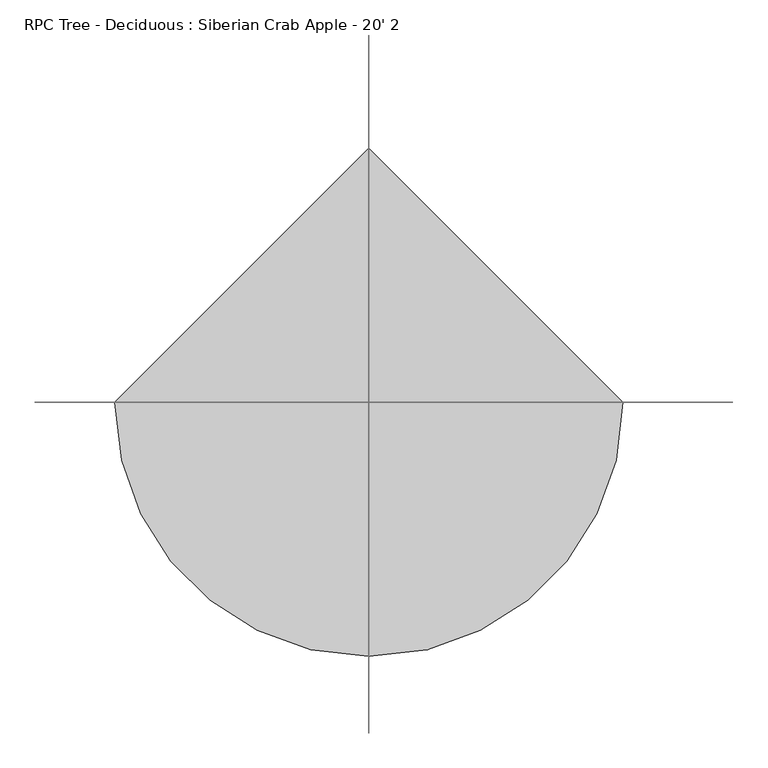
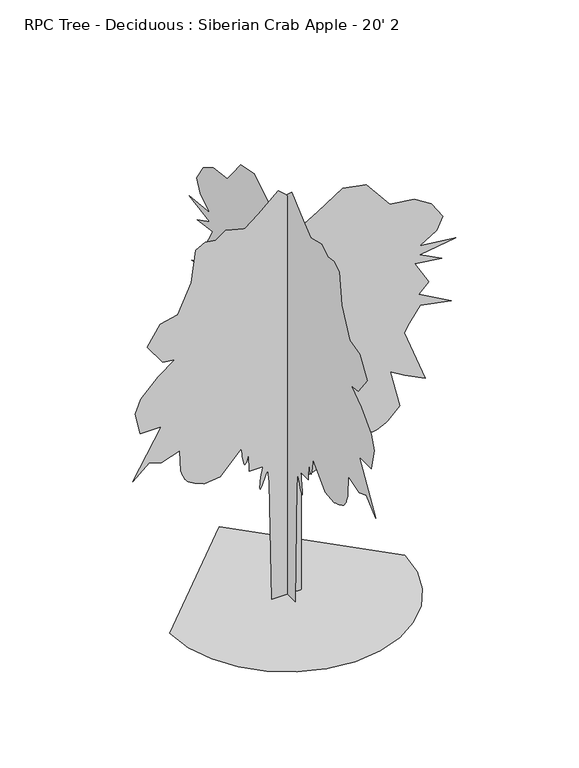
"""IFC4 building model written with IfcOpenShell, lengths in millimetres: geographic element geometry, RPC Tree - Deciduous : Siberian Crab Apple - 20' 2."""

from ifc_helpers import new_model, si_unit, origin, place, context, project, spatial, triangles, source, transform, mapped, element, save


def rpc_tree_deciduous_siberian_crab_apple_20_2_052c092b(model_context):
    return source(origin(), model_context, "Body", "Tessellation", [
        triangles([(-0.5602972, -201.7007698, 0.1401761), (-0.5602953, -233.6267644, 1770.9888485), (-0.560294, -257.4323607, 1961.4323112), (-0.5602928, -281.0760302, 1899.1069004), (-0.5602909, -303.7481383, 1840.3247326), (-0.5602896, -324.477142, 1788.6165516), (-0.560289, -342.2908439, 1747.5319954), (-0.5602877, -356.2177191, 1720.6015171), (-0.5602877, -365.2868239, 1711.3685051), (-0.5602871, -368.5253254, 1723.3764931), (-0.5602871, -367.3690006, 1751.3483322), (-0.5602877, -364.1298451, 1786.8131733), (-0.5602877, -359.1558755, 1828.5264702), (-0.5602883, -352.7938002, 1875.2308868), (-0.560289, -345.3909453, 1925.6881268), (-0.560289, -337.2934018, 1978.6472488), (-0.5602896, -328.8491498, 2032.8510624), (-0.5602782, -519.2951197, 2032.8510624), (-0.5602775, -527.2301368, 2286.7756794), (-0.5602769, -537.409203, 2251.45051), (-0.5602763, -547.4498692, 2218.4176426), (-0.5602763, -557.212391, 2189.9568798), (-0.5602756, -566.5589862, 2168.3731682), (-0.560275, -575.3505644, 2155.95256), (-0.5602744, -583.4474902, 2154.9809624), (-0.5602737, -590.7119087, 2167.7508224), (-0.5602737, -597.2822926, 2191.1633469), (-0.5602731, -603.4360957, 2219.9861515), (-0.5602731, -609.2431904, 2253.3237968), (-0.5602724, -614.7721407, 2290.2745937), (-0.5602724, -620.0934729, 2329.9240631), (-0.5602718, -625.2757147, 2371.3833057), (-0.5602718, -630.3881207, 2413.7443829), (-0.560254, -931.9290173, 2096.3322166), (-0.5602407, -1154.1161819, 2072.5259663), (-0.5602375, -1198.140893, 2089.5313236), (-0.560235, -1241.0543346, 2106.536681), (-0.5602331, -1281.7453102, 2123.5420383), (-0.5602305, -1319.1087273, 2140.5410007), (-0.5602287, -1352.0336071, 2157.5463581), (-0.5602267, -1379.4022854, 2174.5517155), (-0.5602255, -1400.1033474, 2191.5570728), (-0.5602248, -1416.1815811, 2210.4102825), (-0.5602242, -1430.5961082, 2232.5973003), (-0.5602229, -1443.6200226, 2257.5592941), (-0.5602223, -1455.5389172, 2284.7436813), (-0.5602217, -1466.6197815, 2313.5917751), (-0.560221, -1477.1416683, 2343.5511383), (-0.5602204, -1487.3906067, 2374.063084), (-0.5602197, -1503.2656551, 2683.5376534), (-0.5602039, -1765.127869, 2596.2502487), (-0.5601937, -1939.7026783, 2659.7315483), (-0.5601798, -2169.8210449, 2453.4191414), (-0.5602039, -1765.127869, 3135.8495796), (-0.5601861, -2066.6648415, 3135.8495796), (-0.5601816, -2138.0835926, 3453.2552055), (-0.5601867, -2058.7273899, 3651.6364105), (-0.5602013, -1812.7403698, 3905.5610275), (-0.5602153, -1574.6780113, 4080.1419411), (-0.5602051, -1749.2528206, 4103.9419418), (-0.5601925, -1963.5087833, 4397.5478577), (-0.5602032, -1780.9965225, 4683.2161766), (-0.5602178, -1535.0031075, 4738.7598793), (-0.5602293, -1344.5596447, 5151.396611), (-0.5602331, -1281.0784904, 5619.5709412), (-0.5602407, -1146.1786577, 5690.9898376), (-0.5602496, -995.4101715, 5667.1837326), (-0.5602585, -852.5727419, 5770.3396454), (-0.5602744, -582.7769279, 5698.9271439), (-0.5602858, -392.3315758, 5849.6958481), (-0.5603029, -106.6631932, 6095.6895538), (-0.5603163, 115.523381, 5897.3080582), (-0.5603163, 115.523381, 5659.245845), (-0.5603245, 258.3569228, 5476.7401245), (-0.5603366, 456.7385456, 5587.8339249), (-0.5603575, 805.8874374, 5817.9518555), (-0.5603772, 1139.1682571, 5754.4708466), (-0.5603893, 1345.4803734, 5500.5462296), (-0.5603969, 1472.4490768, 5341.8402191), (-0.5604179, 1821.59855, 5294.228009), (-0.5604325, 2067.5919651, 5143.4593048), (-0.560442, 2226.2917259, 4897.4655991), (-0.5604369, 2139.0043213, 4722.8910805), (-0.5604223, 1900.9485031, 4572.1226669), (-0.5604528, 2408.8039867, 4516.5789642), (-0.5604223, 1900.9485031, 4437.2227615), (-0.5604407, 2210.4230724, 4278.5167511), (-0.5604185, 1829.529752, 4326.1292519), (-0.56043, 2027.9108116, 3984.9172302), (-0.5604217, 1885.0797043, 3850.0173248), (-0.560449, 2345.3228325, 3588.1551109), (-0.560423, 1908.8859547, 3675.4425156), (-0.5604134, 1750.1799442, 3461.1928024), (-0.560409, 1678.7611931, 3342.1616959), (-0.5604274, 1980.2983109, 2556.5753448), (-0.5604096, 1686.69879, 2699.4125565), (-0.5603976, 1480.3802788, 2826.374865), (-0.5604052, 1615.2800388, 2270.9070259), (-0.5603956, 1448.6428265, 2104.2696682), (-0.5603937, 1416.3657269, 2085.6895523), (-0.5603918, 1384.3044571, 2067.8777035), (-0.5603899, 1352.6559528, 2051.5900349), (-0.560388, 1321.6297943, 2037.5945229), (-0.5603861, 1291.441666, 2026.6534756), (-0.5603842, 1262.2887943, 2019.5223701), (-0.5603829, 1234.3931133, 2016.9824089), (-0.5603811, 1206.7197298, 2019.0651306), (-0.5603798, 1178.2208879, 2024.894426), (-0.5603779, 1149.0234695, 2033.8479492), (-0.5603759, 1119.2736139, 2045.297105), (-0.5603741, 1089.1046705, 2058.6257973), (-0.5603721, 1058.656311, 2073.1990356), (-0.5603702, 1028.0746748, 2088.3946198), (-0.5603702, 1019.444969, 2098.5293209), (-0.5603696, 1010.0533184, 2108.2448616), (-0.560369, 999.131238, 2117.1284763), (-0.5603677, 985.9231779, 2124.7675449), (-0.5603671, 969.6607985, 2130.7366573), (-0.5603658, 949.5756872, 2134.6229027), (-0.5603645, 924.918544, 2136.0071205), (-0.5603626, 892.850952, 2139.7092201), (-0.5603601, 852.0393442, 2150.0723957), (-0.5603569, 803.9443148, 2165.9919182), (-0.5603537, 750.0199173, 2186.3501232), (-0.5603506, 691.7204235, 2210.041991), (-0.5603467, 630.5036659, 2235.950148), (-0.5603429, 567.8315103, 2262.969429), (-0.5603372, 464.6735264, 2143.9447174), (-0.5603372, 464.6735264, 1945.5636578), (-0.5603404, 520.2190822, 1755.120195), (-0.560329, 329.7743477, 1691.6390408), (-0.560322, 218.6813649, 2001.1073605), (-0.5603233, 220.2409354, 0.0), (-1667.0454838, -6.4e-06, 0.5321514), (-1623.0016605, -381.6984675, 0.5321527), (-1497.5824265, -732.2271807, 0.5321565), (-1300.8143497, -1041.5430387, 0.5321622), (-1042.7559008, -1299.6078827, 0.5321698), (-733.4400427, -1496.3695644, 0.5321793), (-382.9106755, -1621.7887985, 0.5321895), (-1.2126887, -1665.8326218, 0.5322009), (380.4856055, -1621.7887985, 0.5322124), (731.0143187, -1496.3695644, 0.5322225), (1040.3301767, -1299.6014877, 0.532232), (1298.3950207, -1041.5430387, 0.5322396), (1495.1567024, -732.2271807, 0.5322454), (1620.5759365, -381.6978135, 0.5322492), (1664.6197598, 0.0001455, 0.5322505), (-1.2129808, 1665.8326218, 0.5322009), (-223.3549713, 0.0003636, 0.4735541), (-255.2809841, 0.0002642, 1771.3190609), (-279.0865623, 0.0002491, 1961.7689186), (-302.7302317, 0.0002561, 1899.4435078), (-325.4023398, 0.0002559, 1840.654945), (-346.1307258, 0.0002629, 1788.953159), (-363.9444277, 0.0002625, 1747.8622078), (-377.8719206, 0.000262, 1720.9317295), (-386.9404078, 0.0002688, 1711.7051125), (-390.1795269, 0.0002609, 1723.7129551), (-389.0225481, 0.0002601, 1751.6785446), (-385.7840466, 0.0002594, 1787.1433857), (-380.810077, 0.0002586, 1828.8566826), (-374.4480017, 0.0002577, 1875.5673489), (-367.0444928, 0.0002496, 1926.0247341), (-358.9476033, 0.0002487, 1978.9774612), (-350.5033513, 0.0002479, 2033.1812748), (-540.9487035, 0.0002455, 2033.1812748), (-548.8836843, 0.0002299, 2287.1122868), (-559.0634045, 0.00023, 2251.7871174), (-569.1034166, 0.0002374, 2218.747855), (-578.8665925, 0.0002374, 2190.2934872), (-588.2131877, 0.0002372, 2168.7097755), (-597.0041482, 0.0002368, 2156.2827724), (-605.1016917, 0.0002361, 2155.3111748), (-612.3654562, 0.0002351, 2168.0810349), (-618.9364941, 0.0002338, 2191.4935593), (-625.0902609, 0.0002324, 2220.3227589), (-630.8967379, 0.0002308, 2253.6602589), (-636.4244528, 0.0002293, 2290.6046608), (-641.745785, 0.0002276, 2330.2606705), (-646.9273727, 0.0002259, 2371.7135181), (-652.0391247, 0.0002242, 2414.0745953), (-953.5825647, 0.0002432, 2096.668824), (-1175.7697294, 0.0002459, 2072.8625736), (-1219.7944405, 0.0002415, 2089.861536), (-1262.7079548, 0.0002444, 2106.8668934), (-1303.398785, 0.0002403, 2123.8722507), (-1340.7623474, 0.0002364, 2140.8776081), (-1373.6872272, 0.0002403, 2157.8829655), (-1401.0557602, 0.0002373, 2174.8819279), (-1421.7568222, 0.000235, 2191.8872852), (-1437.8350559, 0.000233, 2210.7404949), (-1452.2495831, 0.000231, 2232.9275127), (-1465.2734974, 0.0002291, 2257.8893612), (-1477.1925373, 0.0002346, 2285.0738937), (-1488.2732563, 0.0002327, 2313.9219875), (-1498.7952885, 0.0002309, 2343.8813507), (-1509.0442268, 0.000229, 2374.3995461), (-1524.9192753, 0.0002038, 2683.8742607), (-1786.7814892, 0.0002122, 2596.5868561), (-1961.3561531, 0.0002093, 2660.067865), (-2191.4745197, 0.0002241, 2453.7493538), (-1786.7814892, 0.0001815, 3136.179792), (-2088.3184616, 0.0001838, 3136.179792), (-2159.7372128, 0.0001606, 3453.5918129), (-2080.3810101, 0.0001472, 3651.9730179), (-1834.3938446, 0.0001324, 3905.8976349), (-1596.3316315, 0.0001266, 4080.4721535), (-1770.9062954, 0.0001249, 4104.2785492), (-1985.1624035, 0.0001043, 4397.884465), (-1802.6501427, 9.02e-05, 4683.546389), (-1556.6567276, 8.13e-05, 4739.0964867), (-1366.2132648, 5.68e-05, 5151.7268234), (-1302.7321106, 3.4e-05, 5619.9075485), (-1167.8322052, 2.93e-05, 5691.326445), (-1017.063719, 2.89e-05, 5667.52034), (-874.226362, 2.4e-05, 5770.6762527), (-604.4311295, 2.83e-05, 5699.2573563), (-413.9851233, 1.89e-05, 5850.0260605), (-128.316768, 7e-07, 6096.0197662), (93.8691795, 1.91e-05, 5897.6382706), (93.8691795, 3.35e-05, 5659.5824524), (236.7027213, 4.44e-05, 5477.0703369), (435.0843441, 3.7e-05, 5588.1641373), (784.23389, 1.75e-05, 5818.2884628), (1117.5147097, 2.73e-05, 5754.8074539), (1323.8268986, 3.87e-05, 5500.876442), (1450.7954567, 4.75e-05, 5342.1704315), (1799.9450752, 5.09e-05, 5294.5646164), (2045.9320953, 6.28e-05, 5143.7895172), (2204.6381058, 7.7e-05, 4897.8022064), (2117.3508465, 8.9e-05, 4723.2276878), (1879.294883, 9.41e-05, 4572.4592743), (2387.1503666, 9.74e-05, 4516.9091766), (1879.294883, 0.0001055, 4437.5593689), (2188.7694523, 0.0001087, 4278.8533585), (1807.8761318, 0.0001097, 4326.4655685), (2006.2571915, 0.0001303, 3985.2474426), (1863.4262295, 0.0001361, 3850.3539322), (2323.6693577, 0.0001559, 3588.4853233), (1887.2323345, 0.0001508, 3675.7791229), (1728.5263241, 0.0001576, 3461.5230148), (1657.1077183, 0.0001693, 3342.4983032), (1958.6446907, 0.0002124, 2556.9119522), (1665.0451698, 0.0002038, 2699.7427689), (1458.7266586, 0.0001962, 2826.7050774), (1593.626564, 0.0002321, 2271.2434879), (1426.9892063, 0.0002441, 2104.5998806), (1394.7121067, 0.0002417, 2086.0261597), (1362.6508369, 0.0002467, 2068.2079159), (1331.0023327, 0.0002443, 2051.9264969), (1299.9761742, 0.0002493, 2037.9247353), (1269.7881912, 0.0002469, 2026.983688), (1240.6351742, 0.0002445, 2019.8589775), (1212.7332436, 0.0002494, 2017.3126213), (1185.0661823, 0.0002469, 2019.395343), (1156.5672678, 0.0002441, 2025.2246384), (1127.3699221, 0.0002486, 2034.1781616), (1097.6200665, 0.0002456, 2045.6337124), (1067.451123, 0.0002425, 2058.9560097), (1037.0027636, 0.0002466, 2073.529248), (1006.4210546, 0.0002434, 2088.7312271), (997.7914215, 0.0002424, 2098.8659283), (988.3996983, 0.0002412, 2108.581469), (977.4776905, 0.00024, 2117.4650837), (964.2696304, 0.0002386, 2125.0977573), (948.007251, 0.0002369, 2131.0668697), (927.9221397, 0.0002423, 2134.9529697), (903.2649965, 0.0002401, 2136.3437279), (871.1974045, 0.0002371, 2140.0456821), (830.3857967, 0.0002405, 2150.4090031), (782.2907673, 0.0002357, 2166.3221306), (728.3663698, 0.0002376, 2186.6803356), (670.066876, 0.0002389, 2210.3722034), (608.8494644, 0.0002327, 2236.28661), (546.1773088, 0.0002336, 2263.3060364), (443.0193249, 0.0002425, 2144.2749298), (443.0193249, 0.0002484, 1945.8938702), (498.5654984, 0.0002591, 1755.4504074), (308.1207639, 0.0002658, 1691.9692532), (197.0271634, 0.0002467, 2001.4438225), (198.5867339, 0.0003649, 0.3333907)], [[85, 84, 86], [53, 52, 54], [91, 90, 92], [87, 86, 88], [95, 94, 96], [96, 94, 97], [9, 8, 10], [52, 51, 54], [51, 50, 54], [1, 133, 2], [133, 132, 2], [2, 132, 3], [131, 130, 132], [130, 129, 132], [129, 128, 132], [18, 17, 19], [71, 70, 72], [72, 70, 73], [10, 8, 11], [8, 7, 11], [11, 7, 12], [7, 6, 12], [12, 6, 13], [6, 5, 13], [13, 5, 14], [5, 4, 14], [14, 4, 15], [4, 3, 15], [15, 3, 16], [16, 3, 17], [55, 54, 56], [89, 88, 90], [56, 54, 57], [57, 54, 58], [61, 60, 62], [62, 60, 63], [60, 59, 63], [25, 24, 26], [24, 23, 26], [26, 23, 27], [23, 22, 27], [27, 22, 28], [22, 21, 28], [28, 21, 29], [21, 20, 29], [29, 20, 30], [20, 19, 30], [30, 19, 31], [82, 81, 83], [83, 81, 84], [81, 80, 84], [80, 79, 84], [70, 69, 73], [98, 97, 99], [31, 19, 32], [99, 97, 100], [58, 54, 59], [100, 97, 101], [101, 97, 102], [102, 97, 103], [103, 97, 104], [104, 97, 105], [105, 97, 106], [106, 97, 107], [107, 97, 108], [108, 97, 109], [109, 97, 110], [110, 97, 111], [111, 97, 112], [112, 97, 113], [113, 97, 114], [114, 97, 115], [115, 97, 116], [116, 97, 117], [117, 97, 118], [118, 97, 119], [119, 97, 120], [120, 97, 121], [121, 97, 122], [122, 97, 123], [123, 97, 124], [124, 97, 125], [125, 97, 126], [126, 97, 127], [65, 64, 66], [66, 64, 67], [68, 67, 69], [67, 64, 69], [3, 132, 17], [73, 69, 74], [69, 64, 74], [64, 63, 74], [63, 59, 74], [17, 132, 19], [132, 128, 19], [128, 127, 19], [92, 90, 93], [76, 75, 77], [77, 75, 78], [78, 75, 79], [79, 75, 84], [75, 74, 84], [74, 59, 84], [84, 59, 86], [86, 59, 88], [88, 59, 90], [90, 59, 93], [93, 59, 94], [94, 59, 97], [97, 59, 127], [127, 59, 19], [32, 19, 33], [19, 59, 33], [59, 54, 33], [54, 50, 33], [33, 50, 34], [50, 49, 34], [34, 49, 35], [35, 49, 36], [36, 49, 37], [49, 48, 37], [37, 48, 38], [48, 47, 38], [38, 47, 39], [47, 46, 39], [39, 46, 40], [46, 45, 40], [45, 44, 40], [40, 44, 41], [44, 43, 41], [41, 43, 42], [148, 149, 134], [147, 148, 134], [147, 134, 135], [146, 147, 135], [146, 135, 136], [146, 136, 137], [145, 146, 137], [144, 145, 137], [144, 137, 138], [144, 138, 139], [144, 139, 140], [144, 140, 141], [144, 141, 142], [144, 142, 143], [233, 234, 235], [201, 202, 203], [239, 240, 241], [235, 236, 237], [243, 244, 245], [243, 245, 246], [157, 158, 159], [200, 201, 203], [199, 200, 203], [282, 150, 151], [281, 282, 151], [281, 151, 152], [279, 280, 281], [278, 279, 281], [277, 278, 281], [166, 167, 168], [219, 220, 221], [219, 221, 222], [157, 159, 160], [156, 157, 160], [156, 160, 161], [155, 156, 161], [155, 161, 162], [154, 155, 162], [154, 162, 163], [153, 154, 163], [153, 163, 164], [152, 153, 164], [152, 164, 165], [152, 165, 166], [203, 204, 205], [237, 238, 239], [203, 205, 206], [203, 206, 207], [209, 210, 211], [209, 211, 212], [208, 209, 212], [173, 174, 175], [172, 173, 175], [172, 175, 176], [171, 172, 176], [171, 176, 177], [170, 171, 177], [170, 177, 178], [169, 170, 178], [169, 178, 179], [168, 169, 179], [168, 179, 180], [230, 231, 232], [230, 232, 233], [229, 230, 233], [228, 229, 233], [218, 219, 222], [246, 247, 248], [168, 180, 181], [246, 248, 249], [203, 207, 208], [246, 249, 250], [246, 250, 251], [246, 251, 252], [246, 252, 253], [246, 253, 254], [246, 254, 255], [246, 255, 256], [246, 256, 257], [246, 257, 258], [246, 258, 259], [246, 259, 260], [246, 260, 261], [246, 261, 262], [246, 262, 263], [246, 263, 264], [246, 264, 265], [246, 265, 266], [246, 266, 267], [246, 267, 268], [246, 268, 269], [246, 269, 270], [246, 270, 271], [246, 271, 272], [246, 272, 273], [246, 273, 274], [246, 274, 275], [246, 275, 276], [213, 214, 215], [213, 215, 216], [216, 217, 218], [213, 216, 218], [281, 152, 166], [218, 222, 223], [213, 218, 223], [212, 213, 223], [208, 212, 223], [281, 166, 168], [277, 281, 168], [276, 277, 168], [239, 241, 242], [224, 225, 226], [224, 226, 227], [224, 227, 228], [224, 228, 233], [223, 224, 233], [208, 223, 233], [208, 233, 235], [208, 235, 237], [208, 237, 239], [208, 239, 242], [208, 242, 243], [208, 243, 246], [208, 246, 276], [208, 276, 168], [168, 181, 182], [208, 168, 182], [203, 208, 182], [199, 203, 182], [199, 182, 183], [198, 199, 183], [198, 183, 184], [198, 184, 185], [198, 185, 186], [197, 198, 186], [197, 186, 187], [196, 197, 187], [196, 187, 188], [195, 196, 188], [195, 188, 189], [194, 195, 189], [193, 194, 189], [193, 189, 190], [192, 193, 190], [192, 190, 191]], closed=False),
    ])


if __name__ == "__main__":
    model = new_model("IFC4")
    model_context = context("Model", 3, world=origin())
    ifc_project = project(units=[si_unit("LENGTHUNIT", "METRE", prefix="MILLI")], contexts=[model_context])
    site = spatial("IfcSite", under=ifc_project)
    building = spatial("IfcBuilding", under=site)
    placement = place(None, origin())
    rpc_tree_deciduous_siberian_crab_apple_20_2_shape = rpc_tree_deciduous_siberian_crab_apple_20_2_052c092b(model_context)
    element("IfcGeographicElement", 1, ObjectType="RPC Tree - Deciduous : Siberian Crab Apple - 20' 2", at=placement, inside=building, context=model_context, shape_type="MappedRepresentation", body=[
        mapped(rpc_tree_deciduous_siberian_crab_apple_20_2_shape, transform((0.0, 0.0, 0.0), x_axis=(1.0, 0.0, 0.0), y_axis=(0.0, 1.0, 0.0), z_axis=(0.0, 0.0, 1.0))),
    ])
    save(model, "model.ifc")

# Revit data of these elements
# Project information
#   Project Issue Date = "22/05/20"
#   Project Status = "Project Status"
#   Client Name = "Jacobo Chocron"
#   Project Address = "Enter address here"
#   Project Name = "Spyning cicle"
#   Project Number = "Project Number"
# Type "RPC Tree - Deciduous : Siberian Crab Apple - 20' 2"
#   built-in parameter 1005195 = "RPC-16-G2MF-J1Q0-CAN1-N000-ST1L-LVER-AU"
#   Type Comments = "Siberian Crab Apple"
#   Assembly Code = "G2050500"
#   Height = 6.096 m
#   Default Elevation = 0
